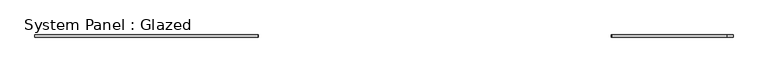
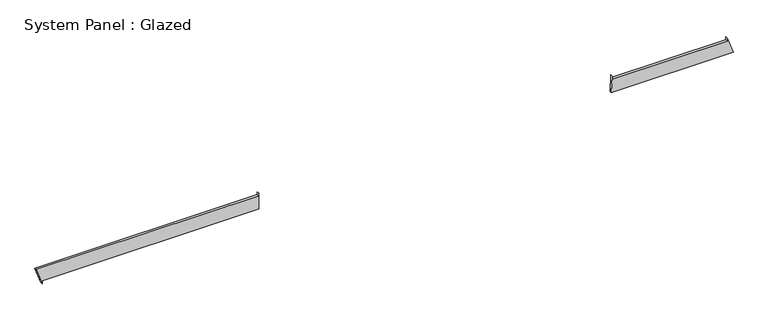
"""IFC4 building model written with IfcOpenShell, lengths in millimetres: plate geometry, System Panel : Glazed."""

from ifc_helpers import new_model, si_unit, frame, origin, place, context, project, spatial, polyline, outline, extrude, source, transform, mapped, element, save


def system_panel_glazed_6b098ca2(model_context):
    return source(origin(), model_context, "Body", "SweptSolid", [
        extrude(outline(polyline([(0.0, -3958.2435347), (35.3553391, -3958.2435347), (35.3553391, -1452.7092746), (234.6359441, -1457.6501), (199.280605, -1457.6494211), (199.2312647, -4027.3171494), (0.0, -3958.2435347)])), frame((0.0, -49.5, 0.0), z_axis=(0.0, 1.0, 0.0), x_axis=(0.0, 0.0, 1.0)), (0.0, 0.0, 1.0), 25.0),
        extrude(outline(polyline([(35.3553391, 2619.8040637), (35.3553391, 4027.3171494), (234.739942, 3958.6129922), (199.3846029, 3958.613671), (199.3590697, 2628.828575), (234.7144087, 2628.8278962), (35.3553391, 2619.8040637)])), frame((0.0, -49.5, 0.0), z_axis=(0.0, 1.0, 0.0), x_axis=(0.0, 0.0, 1.0)), (0.0, 0.0, 1.0), 25.0),
    ])


if __name__ == "__main__":
    model = new_model("IFC4")
    model_context = context("Model", 3, world=origin())
    ifc_project = project(units=[si_unit("LENGTHUNIT", "METRE", prefix="MILLI")], contexts=[model_context])
    site = spatial("IfcSite", under=ifc_project)
    building = spatial("IfcBuilding", under=site)
    placement = place(None, origin())
    system_panel_glazed_shape = system_panel_glazed_6b098ca2(model_context)
    element("IfcPlate", 1, ObjectType="System Panel : Glazed", at=placement, inside=building, context=model_context, shape_type="MappedRepresentation", body=[
        mapped(system_panel_glazed_shape, transform((0.0, 0.0, 0.0), x_axis=(1.0, 0.0, 0.0), y_axis=(0.0, 1.0, 0.0), z_axis=(0.0, 0.0, 1.0))),
    ])
    save(model, "model.ifc")

# Revit data of these elements
# Element 1 (IfcPlate, "System Panel : Glazed")
#   Materials on its faces: "Glass"
# Materials
#   "Glass": class "Glass", colour RGB 218 227 224, transparency 0.85, Description = "Soda Lime Glass", Cost = 0
